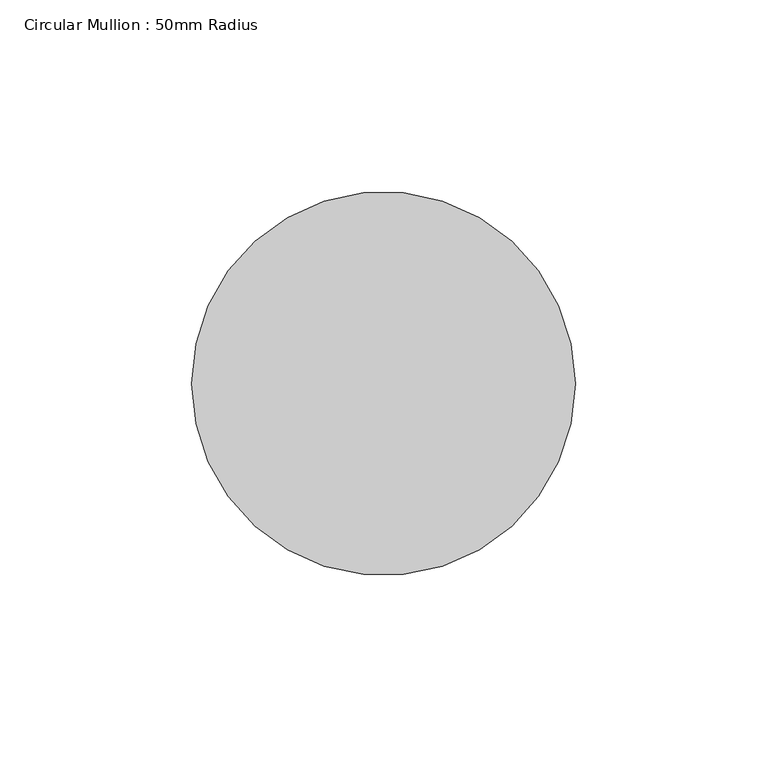
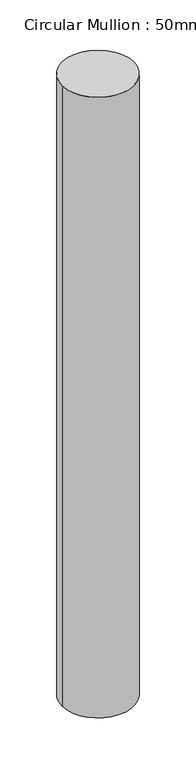
"""IFC4 building model written with IfcOpenShell, lengths in millimetres: member geometry, Circular Mullion : 50mm Radius."""

from ifc_helpers import new_model, si_unit, point, frame, origin, origin_2d, place, context, project, spatial, circle_curve, trimmed, segment, composite_curve, outline, extrude, source, transform, mapped, element, save


def circular_mullion_50mm_radius_1fa6fdaf(model_context):
    return source(origin(), model_context, "Body", "SweptSolid", [
        extrude(outline(composite_curve([segment(trimmed(circle_curve(origin_2d(), 50.0), [point((50.0, 0.0))], [point((-50.0, 0.0))], False, "CARTESIAN"), True, "CONTINUOUS"), segment(trimmed(circle_curve(origin_2d(), 50.0), [point((-50.0, 0.0))], [point((50.0, 0.0))], False, "CARTESIAN"), True, "CONTINUOUS")], self_intersect=False)), frame((0.0, 0.0, -916.0900322), z_axis=(0.0, 0.0, 1.0), x_axis=(1.0, 0.0, 0.0)), (0.0, 0.0, 1.0), 916.0900322),
    ])


if __name__ == "__main__":
    model = new_model("IFC4")
    model_context = context("Model", 3, world=origin())
    ifc_project = project(units=[si_unit("LENGTHUNIT", "METRE", prefix="MILLI")], contexts=[model_context])
    site = spatial("IfcSite", under=ifc_project)
    building = spatial("IfcBuilding", under=site)
    placement = place(None, origin())
    circular_mullion_50mm_radius_shape = circular_mullion_50mm_radius_1fa6fdaf(model_context)
    element("IfcMember", 1, ObjectType="Circular Mullion : 50mm Radius", at=placement, inside=building, context=model_context, shape_type="MappedRepresentation", body=[
        mapped(circular_mullion_50mm_radius_shape, transform((0.0, 0.0, 0.0), x_axis=(1.0, 0.0, 0.0), y_axis=(0.0, 1.0, 0.0), z_axis=(0.0, 0.0, 1.0))),
    ])
    save(model, "model.ifc")

# Revit data of these elements
# Type "Circular Mullion : 50mm Radius"
#   built-in parameter 1007350 = 0.164042 (stored number, unit not read)
# Element 1 (IfcMember, "Circular Mullion : 50mm Radius")
#   Materials on its faces: "Aluminium"
# Materials
#   "Aluminium": class "Metal", colour RGB 247 247 247, transparency 0, Description = "Aluminium 6061", Cost = 0
